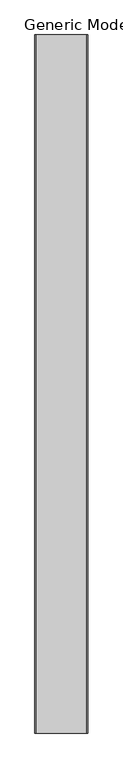
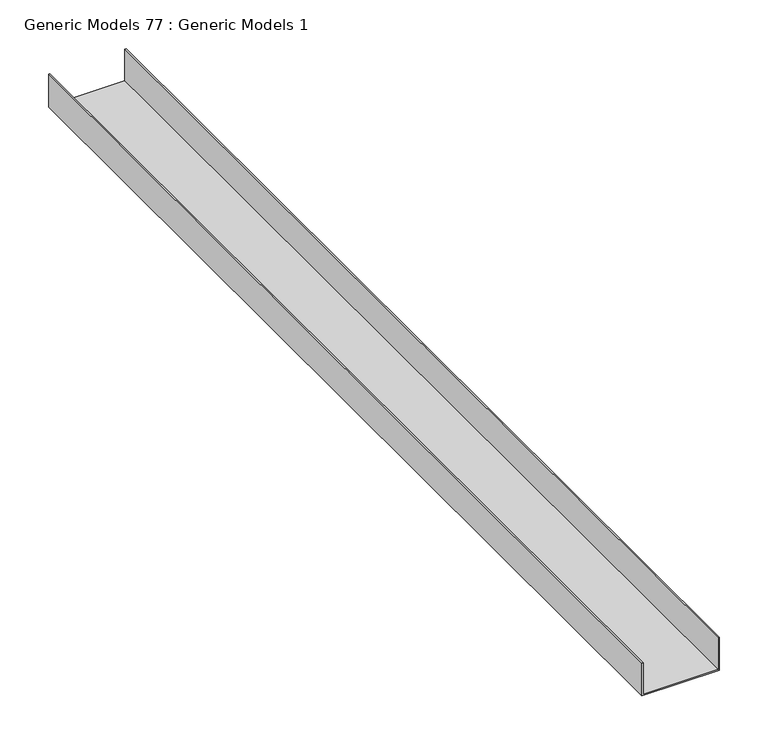
"""IFC4 building model written with IfcOpenShell, lengths in millimetres: proxy geometry, Generic Models 77 : Generic Models 1."""

import ifcopenshell
import ifcopenshell.guid

model = None  # the IFC model being written
_history = None  # IfcOwnerHistory: only IFC2X3 demands one
_inside = {}  # id of a spatial element -> (the spatial element, [elements in it])
_under = {}  # id of a project, library or spatial element -> (it, [spatial elements below it])
_declared = {}  # id of a project -> (the project, [libraries it declares])
_typed = {}  # id of a type object -> (the type object, [elements of that type])
_made_of = {}  # id of a material, layer set ... -> (it, [elements and type objects made of it])


def new_model(schema):
    """Start an empty IFC model of exactly this schema.

    Asked for "IFC4X3", IfcOpenShell would pick the latest addendum, in which some entities
    have other attributes; the version numbers below select the first issue.
    IFC2X3 requires an IfcOwnerHistory on every rooted entity: one is made here for all.
    """
    global model, _history
    if schema == "IFC4X3":
        model = ifcopenshell.file(schema_version=(4, 3, 0, 0))
    else:
        model = ifcopenshell.file(schema=schema)
    _inside.clear()
    _under.clear()
    _declared.clear()
    _typed.clear()
    _made_of.clear()
    _history = None
    if model.schema == "IFC2X3":
        org = make("IfcOrganization", Name="unknown")
        user = make(
            "IfcPersonAndOrganization",
            ThePerson=make("IfcPerson", FamilyName="unknown"),
            TheOrganization=org,
        )
        app = make(
            "IfcApplication",
            ApplicationDeveloper=org,
            Version="unknown",
            ApplicationFullName="unknown",
            ApplicationIdentifier="unknown",
        )
        _history = make(
            "IfcOwnerHistory",
            OwningUser=user,
            OwningApplication=app,
            ChangeAction="ADDED",
            CreationDate=0,
        )
    return model


def make(cls, **values):
    """One entity of the class cls with the attributes given. An attribute that is None is left unset."""
    return model.create_entity(
        cls, **{name: value for name, value in values.items() if value is not None}
    )


def rooted(cls, **values):
    """An entity with a GlobalId (a new one), such as an element, a storey or a relation."""
    return make(cls, GlobalId=ifcopenshell.guid.new(), OwnerHistory=_history, **values)


def si_unit(unit_type, name, prefix=None):
    """IfcSIUnit, for example si_unit("LENGTHUNIT", "METRE", prefix="MILLI")."""
    return make("IfcSIUnit", UnitType=unit_type, Prefix=prefix, Name=name)


def assignment(units):
    """IfcUnitAssignment: the units of a project."""
    return None if units is None else make("IfcUnitAssignment", Units=units)


def point(xyz):
    """IfcCartesianPoint."""
    return None if xyz is None else make("IfcCartesianPoint", Coordinates=xyz)


def direction(xyz):
    """IfcDirection."""
    return None if xyz is None else make("IfcDirection", DirectionRatios=xyz)


def frame(location, z_axis=None, x_axis=None):
    """IfcAxis2Placement3D, a coordinate frame: its origin and axes. An axis left out is left unset."""
    return make(
        "IfcAxis2Placement3D",
        Location=point(location),
        Axis=direction(z_axis),
        RefDirection=direction(x_axis),
    )


def origin():
    """The frame at (0, 0, 0) with its axes left unset."""
    return frame((0.0, 0.0, 0.0))


def place(relative_to, where):
    """IfcLocalPlacement: puts the frame where relative to a parent placement (None: the world)."""
    return make(
        "IfcLocalPlacement", PlacementRelTo=relative_to, RelativePlacement=where
    )


def context(
    kind, dimensions, precision=None, world=None, true_north=None, identifier=None
):
    """IfcGeometricRepresentationContext, for example the 3D "Model" context."""
    return make(
        "IfcGeometricRepresentationContext",
        ContextIdentifier=identifier,
        ContextType=kind,
        CoordinateSpaceDimension=dimensions,
        Precision=precision,
        WorldCoordinateSystem=world,
        TrueNorth=true_north,
    )


def project(units=None, contexts=None):
    """IfcProject with its units and contexts."""
    return rooted(
        "IfcProject",
        Name="project",
        RepresentationContexts=contexts,
        UnitsInContext=assignment(units),
    )


def spatial(cls, under=None, at=None, **own):
    """A site, building, storey or space (cls), placed at a placement, below another one or the project."""
    s = rooted(cls, ObjectPlacement=at, **own)
    if under is not None:
        _under.setdefault(under.id(), (under, []))[1].append(s)
    return s


def polyline(points):
    """IfcPolyline through the points."""
    return make("IfcPolyline", Points=[point(p) for p in points])


def outline(outer, holes=None, kind="AREA"):
    """IfcArbitraryClosedProfileDef: a profile drawn as a closed curve; with holes, ...WithVoids."""
    if holes is None:
        return make("IfcArbitraryClosedProfileDef", ProfileType=kind, OuterCurve=outer)
    return make(
        "IfcArbitraryProfileDefWithVoids",
        ProfileType=kind,
        OuterCurve=outer,
        InnerCurves=holes,
    )


def extrude(swept, where, along, depth):
    """IfcExtrudedAreaSolid: the profile swept, set in the frame where, extruded along a direction by depth."""
    return make(
        "IfcExtrudedAreaSolid",
        SweptArea=swept,
        Position=where,
        ExtrudedDirection=direction(along),
        Depth=depth,
    )


def shape(context_of_items, identifier, shape_type, items):
    """IfcShapeRepresentation: the items that make up one representation, for example the "Body"."""
    return make(
        "IfcShapeRepresentation",
        ContextOfItems=context_of_items,
        RepresentationIdentifier=identifier,
        RepresentationType=shape_type,
        Items=items,
    )


def source(mapping_origin, context_of_items, identifier, shape_type, items):
    """IfcRepresentationMap: a shape defined once, which mapped items show again and again."""
    return make(
        "IfcRepresentationMap",
        MappingOrigin=mapping_origin,
        MappedRepresentation=shape(context_of_items, identifier, shape_type, items),
    )


def transform(
    local_origin,
    x_axis=None,
    y_axis=None,
    z_axis=None,
    scale=None,
    scale2=None,
    scale3=None,
    uniform=True,
):
    """IfcCartesianTransformationOperator3D, or its non-uniform kind. x_axis, y_axis, z_axis: its Axis1, 2, 3."""
    if uniform:
        return make(
            "IfcCartesianTransformationOperator3D",
            Axis1=direction(x_axis),
            Axis2=direction(y_axis),
            LocalOrigin=point(local_origin),
            Scale=scale,
            Axis3=direction(z_axis),
        )
    return make(
        "IfcCartesianTransformationOperator3DnonUniform",
        Axis1=direction(x_axis),
        Axis2=direction(y_axis),
        LocalOrigin=point(local_origin),
        Scale=scale,
        Axis3=direction(z_axis),
        Scale2=scale2,
        Scale3=scale3,
    )


def mapped(mapping_source, mapping_target):
    """IfcMappedItem: shows the shape of a source again, moved by a transform."""
    return make(
        "IfcMappedItem", MappingSource=mapping_source, MappingTarget=mapping_target
    )


def made_of(thing, what):
    """Note that an element or type object is made of a material, layer set ...; save() writes the relation."""
    if what is not None:
        _made_of.setdefault(what.id(), (what, []))[1].append(thing)
    return thing


def element(
    cls,
    number,
    at=None,
    inside=None,
    cuts=None,
    type_object=None,
    material=None,
    context=None,
    identifier="Body",
    shape_type=None,
    held_by="IfcProductDefinitionShape",
    body=None,
    shapes=None,
    **own,
):
    """One element of the class cls, such as IfcWall. Its Tag is "e" and its number.

    at: its placement. inside: the storey or other place that contains it. cuts: it is an
    opening in that element (IfcRelVoidsElement). A single representation is given by context,
    identifier, shape_type and body (its items); several are given by shapes. held_by: the class
    of the entity that holds the representations. save() writes the other relations.
    """
    e = rooted(cls, Tag="e%d" % number, ObjectPlacement=at, **own)
    if body is not None:
        shapes = [shape(context, identifier, shape_type, body)]
    if shapes is not None:
        e.Representation = make(held_by, Representations=shapes)
    if inside is not None:
        _inside.setdefault(inside.id(), (inside, []))[1].append(e)
    if cuts is not None:
        rooted(
            "IfcRelVoidsElement", RelatingBuildingElement=cuts, RelatedOpeningElement=e
        )
    if type_object is not None:
        _typed.setdefault(type_object.id(), (type_object, []))[1].append(e)
    return made_of(e, material)


def aggregate(whole, parts):
    """IfcRelAggregates: a whole, such as a stair, and the parts it consists of."""
    return rooted("IfcRelAggregates", RelatingObject=whole, RelatedObjects=parts)


def save(model, path):
    """Write the relations noted so far, then the file.

    IfcRelAggregates (storeys below a building ...), IfcRelContainedInSpatialStructure (elements
    in a storey), IfcRelDefinesByType, IfcRelAssociatesMaterial and IfcRelDeclares: one each for
    every whole, place, type object, material and project.
    """
    for whole, parts in _under.values():
        aggregate(whole, parts)
    for where, things in _inside.values():
        rooted(
            "IfcRelContainedInSpatialStructure",
            RelatedElements=things,
            RelatingStructure=where,
        )
    for kind, things in _typed.values():
        rooted("IfcRelDefinesByType", RelatedObjects=things, RelatingType=kind)
    for what, things in _made_of.values():
        rooted("IfcRelAssociatesMaterial", RelatedObjects=things, RelatingMaterial=what)
    for by, libraries in _declared.values():
        rooted("IfcRelDeclares", RelatingContext=by, RelatedDefinitions=libraries)
    model.write(path)


def generic_models_77_generic_models_1_8efd1fd8(model_context):
    return source(origin(), model_context, "Body", "SweptSolid", [
        extrude(outline(polyline([(-225.976067, 46935.8735531), (-184.701067, 46935.8735531), (-184.701067, 46934.2860531), (-224.388567, 46934.2860531), (-224.388567, 46845.3860531), (-184.701067, 46845.3860531), (-184.701067, 46843.7985531), (-225.976067, 46843.7985531), (-225.976067, 46935.8735531)])), frame((0.0, 0.0, 0.0), z_axis=(0.0, 1.0, 0.0), x_axis=(0.0, 0.0, 1.0)), (0.0, 0.0, 1.0), 1219.2),
    ])


if __name__ == "__main__":
    model = new_model("IFC4")
    model_context = context("Model", 3, world=origin())
    ifc_project = project(units=[si_unit("LENGTHUNIT", "METRE", prefix="MILLI")], contexts=[model_context])
    site = spatial("IfcSite", under=ifc_project)
    building = spatial("IfcBuilding", under=site)
    placement = place(None, origin())
    generic_models_77_generic_models_1_shape = generic_models_77_generic_models_1_8efd1fd8(model_context)
    element("IfcBuildingElementProxy", 1, Name="Generic Models 77 : Generic Models 1", ObjectType="Generic Models 77 : Generic Models 1", at=placement, inside=building, context=model_context, shape_type="MappedRepresentation", body=[
        mapped(generic_models_77_generic_models_1_shape, transform((0.0, 0.0, 0.0), x_axis=(1.0, 0.0, 0.0), y_axis=(0.0, 1.0, 0.0), z_axis=(0.0, 0.0, 1.0))),
    ])
    save(model, "model.ifc")

# Revit data of these elements
# Element 1 (IfcBuildingElementProxy, "Generic Models 77 : Generic Models 1")
#   Materials on its faces: "METAL RUNNER CHANNEL; FASTEN @ 24\" O.C."
# Materials
#   "METAL RUNNER CHANNEL; FASTEN @ 24\" O.C.": class "Unassigned", colour RGB 210 209 208, transparency 0, Keynote = "M05121300.02", Cost = 0
